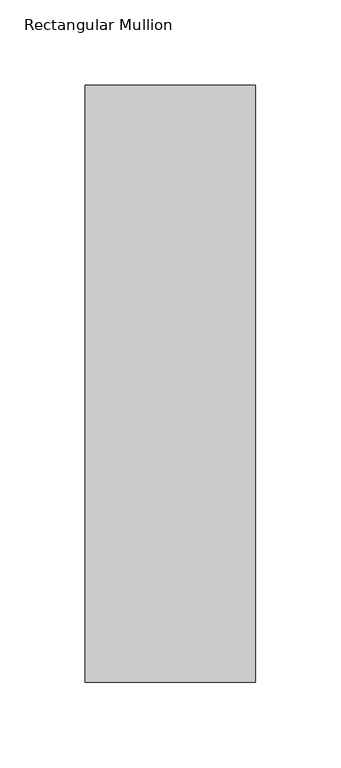
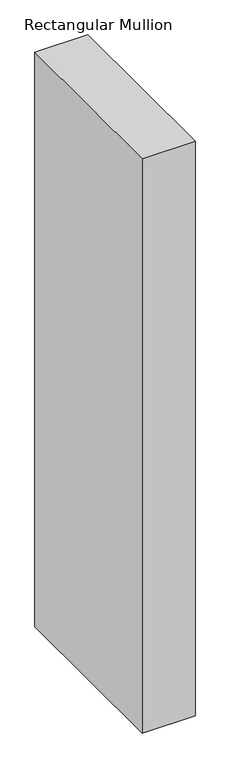
"""IFC4 building model written with IfcOpenShell, lengths in millimetres: member geometry, Rectangular Mullion : WWm-100x350-100mmOffset."""

from ifc_helpers import new_model, si_unit, frame, origin, place, context, project, spatial, polyline, outline, extrude, source, transform, mapped, element, save


def rectangular_mullion_b7f94b0a(model_context):
    return source(origin(), model_context, "Body", "SweptSolid", [
        extrude(outline(polyline([(0.0, 175.0), (0.0, -175.0), (-100.0, -175.0), (-100.0, 175.0), (0.0, 175.0)])), frame((0.0, 0.0, -1145.3542803), z_axis=(0.0, 0.0, 1.0), x_axis=(1.0, 0.0, 0.0)), (0.0, 0.0, 1.0), 1145.3542803),
    ])


if __name__ == "__main__":
    model = new_model("IFC4")
    model_context = context("Model", 3, world=origin())
    ifc_project = project(units=[si_unit("LENGTHUNIT", "METRE", prefix="MILLI")], contexts=[model_context])
    site = spatial("IfcSite", under=ifc_project)
    building = spatial("IfcBuilding", under=site)
    placement = place(None, origin())
    rectangular_mullion_shape = rectangular_mullion_b7f94b0a(model_context)
    element("IfcMember", 1, ObjectType="Rectangular Mullion : WWm-100x350-100mmOffset", at=placement, inside=building, context=model_context, shape_type="MappedRepresentation", body=[
        mapped(rectangular_mullion_shape, transform((0.0, 0.0, 0.0), x_axis=(1.0, 0.0, 0.0), y_axis=(0.0, 1.0, 0.0), z_axis=(0.0, 0.0, 1.0))),
    ])
    save(model, "model.ifc")

# Revit data of these elements
# Type "Rectangular Mullion : WWm-100x350-100mmOffset"
#   built-in parameter 1007304 = 1.14829 (stored number, unit not read)
#   built-in parameter 1007301 = 0.164042 (stored number, unit not read)
#   built-in parameter 1007300 = 0.164042 (stored number, unit not read)
# Element 1 (IfcMember, "Rectangular Mullion : WWm-100x350-100mmOffset")
#   Materials on its faces: "WW-EC-RGB-Mullion"
# Materials
#   "WW-EC-RGB-Mullion": class "Generic", colour RGB 255 255 255, transparency 0, Comments = "If region requests black mullions, switch asset color to RGB 25-25-25", Description = "Generic Color", Cost = 0
